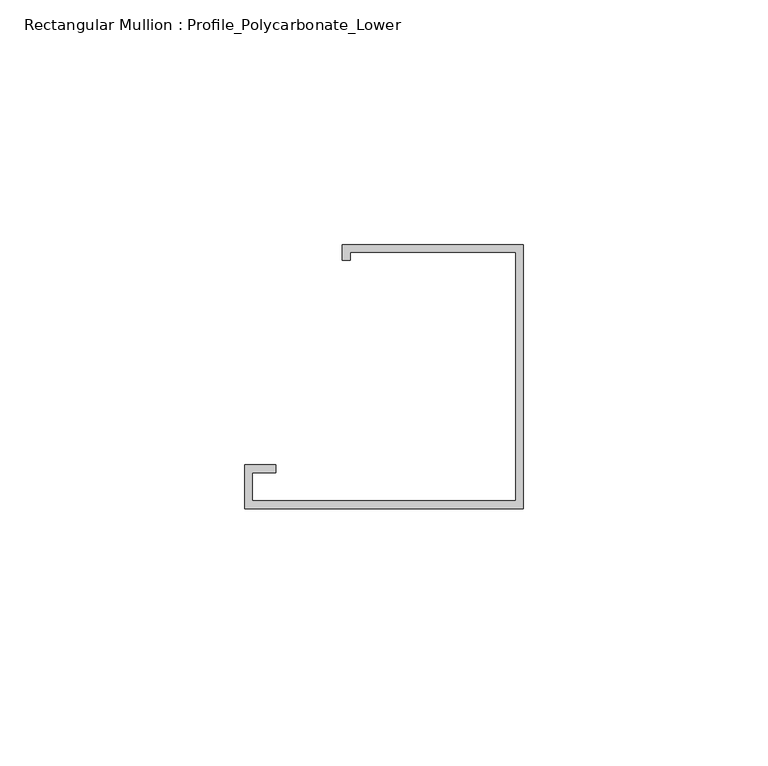
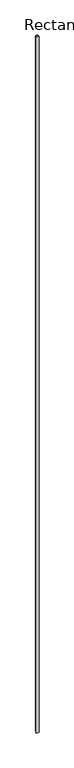
"""IFC4 building model written with IfcOpenShell, lengths in millimetres: member geometry, Rectangular Mullion : Profile_Polycarbonate_Lower."""

from ifc_helpers import new_model, si_unit, frame, origin, place, context, project, spatial, polyline, outline, extrude, source, transform, mapped, element, save


def rectangular_mullion_profile_polycarbonate_lower_16d1c686(model_context):
    return source(origin(), model_context, "Body", "SweptSolid", [
        extrude(outline(polyline([(0.0, -28.984575), (-56.9976, -28.984575), (-56.9976, -19.992975), (-50.6476, -19.992975), (-50.6476, -21.580475), (-55.4101, -21.580475), (-55.4101, -27.397075), (-1.5875, -27.397075), (-1.5875, 23.428325), (-35.3949, 23.428325), (-35.3949, 21.840825), (-36.9824, 21.840825), (-36.9824, 25.015825), (0.0, 25.015825), (0.0, -28.984575)])), frame((0.0, 0.0, -14432.1149), z_axis=(0.0, 0.0, 1.0), x_axis=(1.0, 0.0, 0.0)), (0.0, 0.0, 1.0), 14432.1149),
    ])


if __name__ == "__main__":
    model = new_model("IFC4")
    model_context = context("Model", 3, world=origin())
    ifc_project = project(units=[si_unit("LENGTHUNIT", "METRE", prefix="MILLI")], contexts=[model_context])
    site = spatial("IfcSite", under=ifc_project)
    building = spatial("IfcBuilding", under=site)
    placement = place(None, origin())
    rectangular_mullion_profile_polycarbonate_lower_shape = rectangular_mullion_profile_polycarbonate_lower_16d1c686(model_context)
    element("IfcMember", 1, ObjectType="Rectangular Mullion : Profile_Polycarbonate_Lower", at=placement, inside=building, context=model_context, shape_type="MappedRepresentation", body=[
        mapped(rectangular_mullion_profile_polycarbonate_lower_shape, transform((0.0, 0.0, 0.0), x_axis=(1.0, 0.0, 0.0), y_axis=(0.0, 1.0, 0.0), z_axis=(0.0, 0.0, 1.0))),
    ])
    save(model, "model.ifc")

# Revit data of these elements
# Type "Rectangular Mullion : Profile_Polycarbonate_Lower"
#   built-in parameter 1007322 = 0.177167 (stored number, unit not read)
#   built-in parameter 1007321 = 0 (stored number, unit not read)
#   built-in parameter 1007320 = 0.00520833 (stored number, unit not read)
